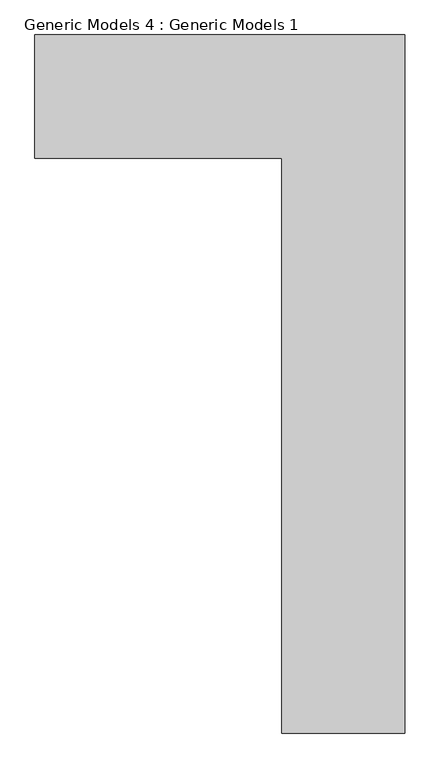
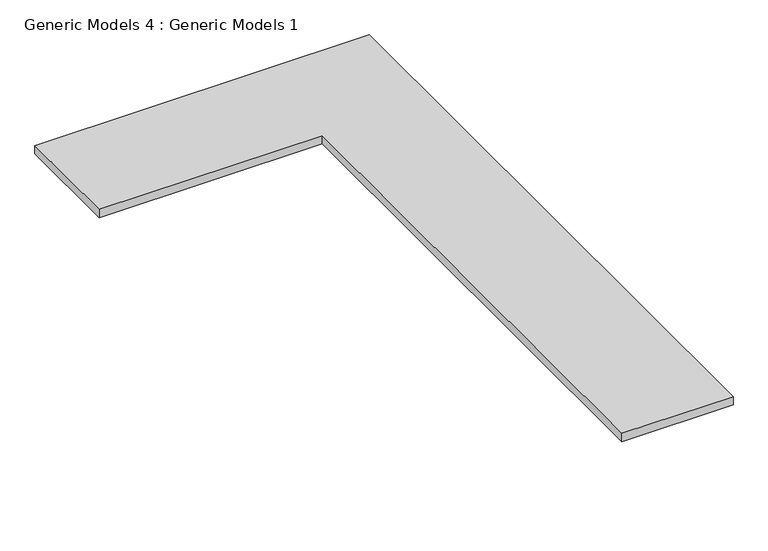
"""IFC4 building model written with IfcOpenShell, lengths in millimetres: furniture geometry, Generic Models 4 : Generic Models 1."""

import ifcopenshell
import ifcopenshell.guid

model = None  # the IFC model being written
_history = None  # IfcOwnerHistory: only IFC2X3 demands one
_inside = {}  # id of a spatial element -> (the spatial element, [elements in it])
_under = {}  # id of a project, library or spatial element -> (it, [spatial elements below it])
_declared = {}  # id of a project -> (the project, [libraries it declares])
_typed = {}  # id of a type object -> (the type object, [elements of that type])
_made_of = {}  # id of a material, layer set ... -> (it, [elements and type objects made of it])


def new_model(schema):
    """Start an empty IFC model of exactly this schema.

    Asked for "IFC4X3", IfcOpenShell would pick the latest addendum, in which some entities
    have other attributes; the version numbers below select the first issue.
    IFC2X3 requires an IfcOwnerHistory on every rooted entity: one is made here for all.
    """
    global model, _history
    if schema == "IFC4X3":
        model = ifcopenshell.file(schema_version=(4, 3, 0, 0))
    else:
        model = ifcopenshell.file(schema=schema)
    _inside.clear()
    _under.clear()
    _declared.clear()
    _typed.clear()
    _made_of.clear()
    _history = None
    if model.schema == "IFC2X3":
        org = make("IfcOrganization", Name="unknown")
        user = make(
            "IfcPersonAndOrganization",
            ThePerson=make("IfcPerson", FamilyName="unknown"),
            TheOrganization=org,
        )
        app = make(
            "IfcApplication",
            ApplicationDeveloper=org,
            Version="unknown",
            ApplicationFullName="unknown",
            ApplicationIdentifier="unknown",
        )
        _history = make(
            "IfcOwnerHistory",
            OwningUser=user,
            OwningApplication=app,
            ChangeAction="ADDED",
            CreationDate=0,
        )
    return model


def make(cls, **values):
    """One entity of the class cls with the attributes given. An attribute that is None is left unset."""
    return model.create_entity(
        cls, **{name: value for name, value in values.items() if value is not None}
    )


def rooted(cls, **values):
    """An entity with a GlobalId (a new one), such as an element, a storey or a relation."""
    return make(cls, GlobalId=ifcopenshell.guid.new(), OwnerHistory=_history, **values)


def si_unit(unit_type, name, prefix=None):
    """IfcSIUnit, for example si_unit("LENGTHUNIT", "METRE", prefix="MILLI")."""
    return make("IfcSIUnit", UnitType=unit_type, Prefix=prefix, Name=name)


def assignment(units):
    """IfcUnitAssignment: the units of a project."""
    return None if units is None else make("IfcUnitAssignment", Units=units)


def point(xyz):
    """IfcCartesianPoint."""
    return None if xyz is None else make("IfcCartesianPoint", Coordinates=xyz)


def direction(xyz):
    """IfcDirection."""
    return None if xyz is None else make("IfcDirection", DirectionRatios=xyz)


def frame(location, z_axis=None, x_axis=None):
    """IfcAxis2Placement3D, a coordinate frame: its origin and axes. An axis left out is left unset."""
    return make(
        "IfcAxis2Placement3D",
        Location=point(location),
        Axis=direction(z_axis),
        RefDirection=direction(x_axis),
    )


def origin():
    """The frame at (0, 0, 0) with its axes left unset."""
    return frame((0.0, 0.0, 0.0))


def place(relative_to, where):
    """IfcLocalPlacement: puts the frame where relative to a parent placement (None: the world)."""
    return make(
        "IfcLocalPlacement", PlacementRelTo=relative_to, RelativePlacement=where
    )


def context(
    kind, dimensions, precision=None, world=None, true_north=None, identifier=None
):
    """IfcGeometricRepresentationContext, for example the 3D "Model" context."""
    return make(
        "IfcGeometricRepresentationContext",
        ContextIdentifier=identifier,
        ContextType=kind,
        CoordinateSpaceDimension=dimensions,
        Precision=precision,
        WorldCoordinateSystem=world,
        TrueNorth=true_north,
    )


def project(units=None, contexts=None):
    """IfcProject with its units and contexts."""
    return rooted(
        "IfcProject",
        Name="project",
        RepresentationContexts=contexts,
        UnitsInContext=assignment(units),
    )


def spatial(cls, under=None, at=None, **own):
    """A site, building, storey or space (cls), placed at a placement, below another one or the project."""
    s = rooted(cls, ObjectPlacement=at, **own)
    if under is not None:
        _under.setdefault(under.id(), (under, []))[1].append(s)
    return s


def polyline(points):
    """IfcPolyline through the points."""
    return make("IfcPolyline", Points=[point(p) for p in points])


def outline(outer, holes=None, kind="AREA"):
    """IfcArbitraryClosedProfileDef: a profile drawn as a closed curve; with holes, ...WithVoids."""
    if holes is None:
        return make("IfcArbitraryClosedProfileDef", ProfileType=kind, OuterCurve=outer)
    return make(
        "IfcArbitraryProfileDefWithVoids",
        ProfileType=kind,
        OuterCurve=outer,
        InnerCurves=holes,
    )


def extrude(swept, where, along, depth):
    """IfcExtrudedAreaSolid: the profile swept, set in the frame where, extruded along a direction by depth."""
    return make(
        "IfcExtrudedAreaSolid",
        SweptArea=swept,
        Position=where,
        ExtrudedDirection=direction(along),
        Depth=depth,
    )


def shape(context_of_items, identifier, shape_type, items):
    """IfcShapeRepresentation: the items that make up one representation, for example the "Body"."""
    return make(
        "IfcShapeRepresentation",
        ContextOfItems=context_of_items,
        RepresentationIdentifier=identifier,
        RepresentationType=shape_type,
        Items=items,
    )


def source(mapping_origin, context_of_items, identifier, shape_type, items):
    """IfcRepresentationMap: a shape defined once, which mapped items show again and again."""
    return make(
        "IfcRepresentationMap",
        MappingOrigin=mapping_origin,
        MappedRepresentation=shape(context_of_items, identifier, shape_type, items),
    )


def transform(
    local_origin,
    x_axis=None,
    y_axis=None,
    z_axis=None,
    scale=None,
    scale2=None,
    scale3=None,
    uniform=True,
):
    """IfcCartesianTransformationOperator3D, or its non-uniform kind. x_axis, y_axis, z_axis: its Axis1, 2, 3."""
    if uniform:
        return make(
            "IfcCartesianTransformationOperator3D",
            Axis1=direction(x_axis),
            Axis2=direction(y_axis),
            LocalOrigin=point(local_origin),
            Scale=scale,
            Axis3=direction(z_axis),
        )
    return make(
        "IfcCartesianTransformationOperator3DnonUniform",
        Axis1=direction(x_axis),
        Axis2=direction(y_axis),
        LocalOrigin=point(local_origin),
        Scale=scale,
        Axis3=direction(z_axis),
        Scale2=scale2,
        Scale3=scale3,
    )


def mapped(mapping_source, mapping_target):
    """IfcMappedItem: shows the shape of a source again, moved by a transform."""
    return make(
        "IfcMappedItem", MappingSource=mapping_source, MappingTarget=mapping_target
    )


def made_of(thing, what):
    """Note that an element or type object is made of a material, layer set ...; save() writes the relation."""
    if what is not None:
        _made_of.setdefault(what.id(), (what, []))[1].append(thing)
    return thing


def element(
    cls,
    number,
    at=None,
    inside=None,
    cuts=None,
    type_object=None,
    material=None,
    context=None,
    identifier="Body",
    shape_type=None,
    held_by="IfcProductDefinitionShape",
    body=None,
    shapes=None,
    **own,
):
    """One element of the class cls, such as IfcWall. Its Tag is "e" and its number.

    at: its placement. inside: the storey or other place that contains it. cuts: it is an
    opening in that element (IfcRelVoidsElement). A single representation is given by context,
    identifier, shape_type and body (its items); several are given by shapes. held_by: the class
    of the entity that holds the representations. save() writes the other relations.
    """
    e = rooted(cls, Tag="e%d" % number, ObjectPlacement=at, **own)
    if body is not None:
        shapes = [shape(context, identifier, shape_type, body)]
    if shapes is not None:
        e.Representation = make(held_by, Representations=shapes)
    if inside is not None:
        _inside.setdefault(inside.id(), (inside, []))[1].append(e)
    if cuts is not None:
        rooted(
            "IfcRelVoidsElement", RelatingBuildingElement=cuts, RelatedOpeningElement=e
        )
    if type_object is not None:
        _typed.setdefault(type_object.id(), (type_object, []))[1].append(e)
    return made_of(e, material)


def aggregate(whole, parts):
    """IfcRelAggregates: a whole, such as a stair, and the parts it consists of."""
    return rooted("IfcRelAggregates", RelatingObject=whole, RelatedObjects=parts)


def save(model, path):
    """Write the relations noted so far, then the file.

    IfcRelAggregates (storeys below a building ...), IfcRelContainedInSpatialStructure (elements
    in a storey), IfcRelDefinesByType, IfcRelAssociatesMaterial and IfcRelDeclares: one each for
    every whole, place, type object, material and project.
    """
    for whole, parts in _under.values():
        aggregate(whole, parts)
    for where, things in _inside.values():
        rooted(
            "IfcRelContainedInSpatialStructure",
            RelatedElements=things,
            RelatingStructure=where,
        )
    for kind, things in _typed.values():
        rooted("IfcRelDefinesByType", RelatedObjects=things, RelatingType=kind)
    for what, things in _made_of.values():
        rooted("IfcRelAssociatesMaterial", RelatedObjects=things, RelatingMaterial=what)
    for by, libraries in _declared.values():
        rooted("IfcRelDeclares", RelatingContext=by, RelatedDefinitions=libraries)
    model.write(path)


def generic_models_4_generic_models_1_c34984c3(model_context):
    return source(origin(), model_context, "Body", "SweptSolid", [
        extrude(outline(polyline([(32425.9652986, -18796.4330088), (32425.9652986, -22396.8830088), (31790.9652986, -22396.8830088), (31790.9652986, -19431.4330088), (30517.7152986, -19431.4330088), (30517.7152986, -18796.4330088), (32425.9652986, -18796.4330088)])), frame((0.0, 0.0, 4419.6), z_axis=(0.0, 0.0, 1.0), x_axis=(1.0, 0.0, 0.0)), (0.0, 0.0, 1.0), 50.8),
    ])


if __name__ == "__main__":
    model = new_model("IFC4")
    model_context = context("Model", 3, world=origin())
    ifc_project = project(units=[si_unit("LENGTHUNIT", "METRE", prefix="MILLI")], contexts=[model_context])
    site = spatial("IfcSite", under=ifc_project)
    building = spatial("IfcBuilding", under=site)
    placement = place(None, origin())
    generic_models_4_generic_models_1_shape = generic_models_4_generic_models_1_c34984c3(model_context)
    element("IfcFurniture", 1, ObjectType="Generic Models 4 : Generic Models 1", at=placement, inside=building, context=model_context, shape_type="MappedRepresentation", body=[
        mapped(generic_models_4_generic_models_1_shape, transform((0.0, 0.0, 0.0), x_axis=(1.0, 0.0, 0.0), y_axis=(0.0, 1.0, 0.0), z_axis=(0.0, 0.0, 1.0))),
    ])
    save(model, "model.ifc")

# Revit data of these elements
# Element 1 (IfcFurniture, "Generic Models 4 : Generic Models 1")
#   Materials on its faces: "casework"
# Materials
#   "casework": class "Generic", colour RGB 209 209 209, transparency 0, Cost = 0
